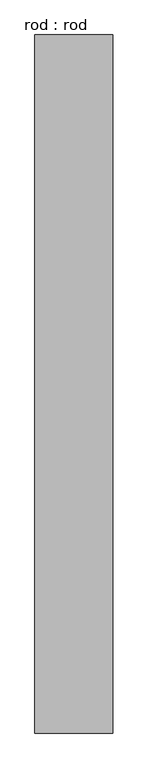
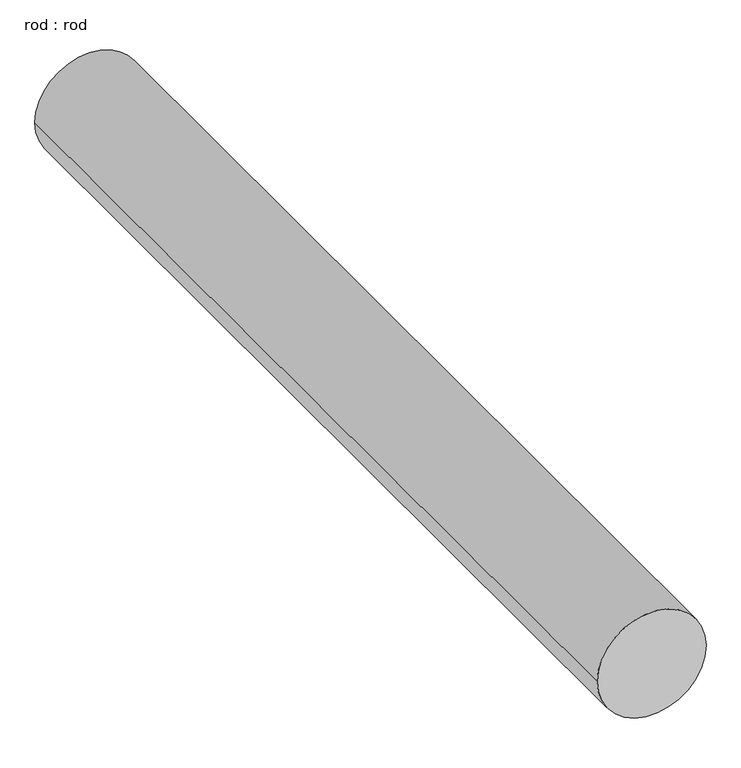
"""IFC4 building model written with IfcOpenShell, lengths in millimetres: proxy geometry, rod : rod."""

from ifc_helpers import new_model, si_unit, point, frame, frame_2d, origin, place, context, project, spatial, circle_curve, trimmed, segment, composite_curve, outline, extrude, source, transform, mapped, element, save


def rod_rod_ca87fe96(model_context):
    return source(origin(), model_context, "Body", "SweptSolid", [
        extrude(outline(composite_curve([segment(trimmed(circle_curve(frame_2d((0.0108462, 0.0)), 200.0), [point((0.0108462, 200.0))], [point((0.0108462, -200.0))], False, "CARTESIAN"), True, "CONTINUOUS"), segment(trimmed(circle_curve(frame_2d((0.0108462, 0.0)), 200.0), [point((0.0108462, -200.0))], [point((0.0108462, 200.0))], False, "CARTESIAN"), True, "CONTINUOUS")], self_intersect=False)), frame((0.0, 2303.4429011, 0.0), z_axis=(0.0, 1.0, 0.0), x_axis=(0.0, 0.0, 1.0)), (0.0, 0.0, 1.0), 3578.5714286),
    ])


if __name__ == "__main__":
    model = new_model("IFC4")
    model_context = context("Model", 3, world=origin())
    ifc_project = project(units=[si_unit("LENGTHUNIT", "METRE", prefix="MILLI")], contexts=[model_context])
    site = spatial("IfcSite", under=ifc_project)
    building = spatial("IfcBuilding", under=site)
    placement = place(None, origin())
    rod_rod_shape = rod_rod_ca87fe96(model_context)
    element("IfcBuildingElementProxy", 1, Name="rod : rod", ObjectType="rod : rod", at=placement, inside=building, context=model_context, shape_type="MappedRepresentation", body=[
        mapped(rod_rod_shape, transform((0.0, 0.0, 0.0), x_axis=(1.0, 0.0, 0.0), y_axis=(0.0, 1.0, 0.0), z_axis=(0.0, 0.0, 1.0))),
    ])
    save(model, "model.ifc")

# Revit data of these elements
# Type "rod : rod"
#   Default Elevation = 0
